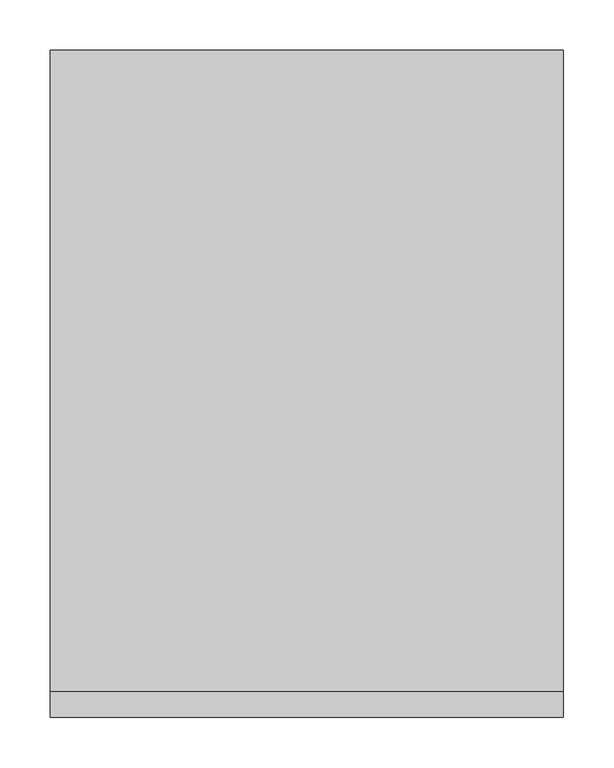
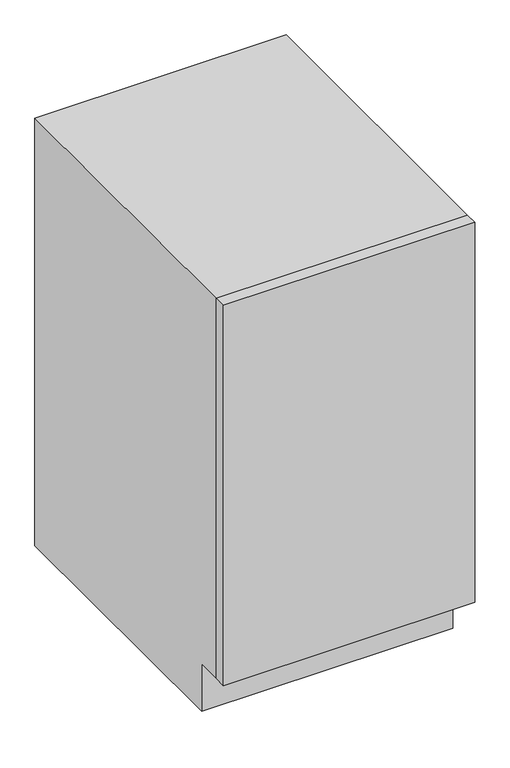
"""IFC4 building model written with IfcOpenShell, lengths in millimetres: furniture geometry, OD_CW_Base Cabinet : OD_CW_Base Cabinet."""

from ifc_helpers import new_model, si_unit, frame, origin, place, context, project, spatial, polyline, outline, extrude, source, transform, mapped, element, save


def furniture_06f6e5f2(model_context):
    return source(origin(), model_context, "Body", "SweptSolid", [
        extrude(outline(polyline([(18.7377049, -25.4), (526.7377049, -25.4), (526.7377049, -50.8), (18.7377049, -50.8), (18.7377049, -25.4)])), frame((0.0, 0.0, 101.6), z_axis=(0.0, 0.0, 1.0), x_axis=(1.0, 0.0, 0.0)), (0.0, 0.0, 1.0), 812.8),
        extrude(outline(polyline([(-25.4, 914.4), (609.6, 914.4), (609.6, 0.0), (25.4, 0.0), (25.4, 101.6), (-25.4, 101.6), (-25.4, 914.4)])), frame((18.7377049, 0.0, 0.0), z_axis=(1.0, 0.0, 0.0), x_axis=(0.0, 1.0, 0.0)), (0.0, 0.0, 1.0), 508.0),
    ])


if __name__ == "__main__":
    model = new_model("IFC4")
    model_context = context("Model", 3, world=origin())
    ifc_project = project(units=[si_unit("LENGTHUNIT", "METRE", prefix="MILLI")], contexts=[model_context])
    site = spatial("IfcSite", under=ifc_project)
    building = spatial("IfcBuilding", under=site)
    placement = place(None, origin())
    furniture_shape = furniture_06f6e5f2(model_context)
    element("IfcFurniture", 1, ObjectType="OD_CW_Base Cabinet : OD_CW_Base Cabinet", at=placement, inside=building, context=model_context, shape_type="MappedRepresentation", body=[
        mapped(furniture_shape, transform((0.0, 0.0, 0.0), x_axis=(1.0, 0.0, 0.0), y_axis=(0.0, 1.0, 0.0), z_axis=(0.0, 0.0, 1.0))),
    ])
    save(model, "model.ifc")

# Revit data of these elements
# Type "OD_CW_Base Cabinet : OD_CW_Base Cabinet"
#   OD_CW_Width [instance default] = 2' - 10"
#   OD_CW_Length [instance default] = 8' - 0"
#   OD_CW_Height [instance default] = 2' - 3"
#   Depth = 2' - 0"
#   Height = 3' - 0"
#   Width = 4' - 0"
#   OD_CW_Material_Front Panel [instance default] = none
#   OD_CW_Material_Body [instance default] = none
# Element 1 (IfcFurniture, "OD_CW_Base Cabinet : OD_CW_Base Cabinet")
#   OD_CW_Width = 2' - 2"
#   OD_CW_Length = 1' - 8"
#   OD_CW_Height = 3' - 0"
#   OD_CW_Material_Body = SPEED RACK
#   Materials on its faces: "SPEED RACK", "CASEWORK"
# Materials
#   "SPEED RACK": class "Generic", colour RGB 187 187 187, transparency 0, Cost = 0
#   "CASEWORK": class "Generic", colour RGB 181 181 181, transparency 0, Cost = 0
